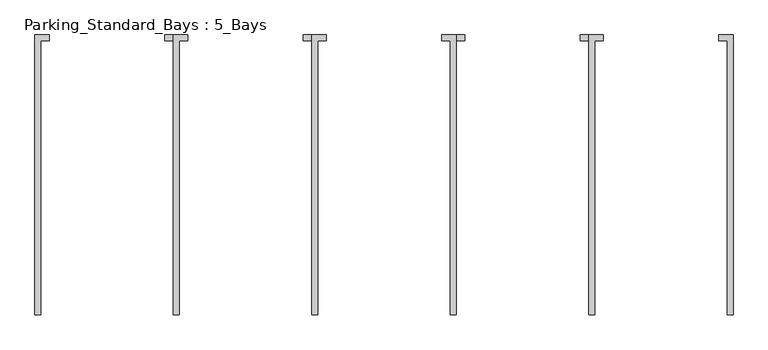
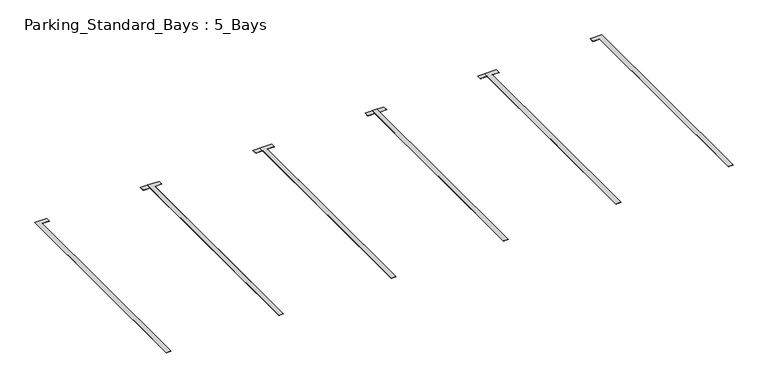
"""IFC4 building model written with IfcOpenShell, lengths in millimetres: proxy geometry, Parking_Standard_Bays : 5_Bays."""

from ifc_helpers import new_model, si_unit, origin, origin_with_axes, place, context, project, spatial, polyline, outline, extrude, source, transform, mapped, element, save


def parking_standard_bays_5_bays_00e1b54b(model_context):
    return source(origin(), model_context, "Body", "SweptSolid", [
        extrude(outline(polyline([(11950.0, 0.0), (11950.0, 4750.0), (11800.0, 4750.0), (11800.0, 4850.0), (12050.0, 4850.0), (12050.0, 0.0), (11950.0, 0.0)])), origin_with_axes(), (0.0, 0.0, 1.0), 3.175),
        extrude(outline(polyline([(9550.0, 0.0), (9550.0, 4850.0), (9800.0, 4850.0), (9800.0, 4750.0), (9650.0, 4750.0), (9650.0, 0.0), (9550.0, 0.0)])), origin_with_axes(), (0.0, 0.0, 1.0), 3.175),
        extrude(outline(polyline([(7150.0, 0.0), (7150.0, 4750.0), (7000.0, 4750.0), (7000.0, 4850.0), (7250.0, 4850.0), (7250.0, 0.0), (7150.0, 0.0)])), origin_with_axes(), (0.0, 0.0, 1.0), 3.175),
        extrude(outline(polyline([(4750.0, 0.0), (4750.0, 4850.0), (5000.0, 4850.0), (5000.0, 4750.0), (4850.0, 4750.0), (4850.0, 0.0), (4750.0, 0.0)])), origin_with_axes(), (0.0, 0.0, 1.0), 3.175),
        extrude(outline(polyline([(4750.0, 0.0), (4750.0, 4750.0), (4600.0, 4750.0), (4600.0, 4850.0), (4850.0, 4850.0), (4850.0, 0.0), (4750.0, 0.0)])), origin_with_axes(), (0.0, 0.0, 1.0), 3.175),
        extrude(outline(polyline([(2350.0, 0.0), (2350.0, 4850.0), (2600.0, 4850.0), (2600.0, 4750.0), (2450.0, 4750.0), (2450.0, 0.0), (2350.0, 0.0)])), origin_with_axes(), (0.0, 0.0, 1.0), 3.175),
        extrude(outline(polyline([(9550.0, 0.0), (9550.0, 4750.0), (9400.0, 4750.0), (9400.0, 4850.0), (9650.0, 4850.0), (9650.0, 0.0), (9550.0, 0.0)])), origin_with_axes(), (0.0, 0.0, 1.0), 3.175),
        extrude(outline(polyline([(7150.0, 0.0), (7150.0, 4850.0), (7400.0, 4850.0), (7400.0, 4750.0), (7250.0, 4750.0), (7250.0, 0.0), (7150.0, 0.0)])), origin_with_axes(), (0.0, 0.0, 1.0), 3.175),
        extrude(outline(polyline([(2350.0, 0.0), (2350.0, 4750.0), (2200.0, 4750.0), (2200.0, 4850.0), (2450.0, 4850.0), (2450.0, 0.0), (2350.0, 0.0)])), origin_with_axes(), (0.0, 0.0, 1.0), 3.175),
        extrude(outline(polyline([(-50.0, 0.0), (-50.0, 4850.0), (200.0, 4850.0), (200.0, 4750.0), (50.0, 4750.0), (50.0, 0.0), (-50.0, 0.0)])), origin_with_axes(), (0.0, 0.0, 1.0), 3.175),
    ])


if __name__ == "__main__":
    model = new_model("IFC4")
    model_context = context("Model", 3, world=origin())
    ifc_project = project(units=[si_unit("LENGTHUNIT", "METRE", prefix="MILLI")], contexts=[model_context])
    site = spatial("IfcSite", under=ifc_project)
    building = spatial("IfcBuilding", under=site)
    placement = place(None, origin())
    parking_standard_bays_5_bays_shape = parking_standard_bays_5_bays_00e1b54b(model_context)
    element("IfcBuildingElementProxy", 1, Name="Parking_Standard_Bays : 5_Bays", ObjectType="Parking_Standard_Bays : 5_Bays", at=placement, inside=building, context=model_context, shape_type="MappedRepresentation", body=[
        mapped(parking_standard_bays_5_bays_shape, transform((0.0, 0.0, 0.0), x_axis=(1.0, 0.0, 0.0), y_axis=(0.0, 1.0, 0.0), z_axis=(0.0, 0.0, 1.0))),
    ])
    save(model, "model.ifc")

# Revit data of these elements
# Type "Parking_Standard_Bays : 5_Bays"
#   Keynote = "Q22/185"
#   Length [instance default] = 14400 mm
#   Bay Width = 2400 mm
#   Bay Length = 4800 mm
#   No of Bays in Array [instance default] = 5
#   No of Bays [instance default] = 6
#   Material - White Lining = Paint - White Lining
# Element 1 (IfcBuildingElementProxy, "Parking_Standard_Bays : 5_Bays")
#   Length = 12000 mm
#   No of Bays in Array = 4
#   No of Bays = 5
#   Materials on its faces: "Paint - White Lining"
# Materials
#   "Paint - White Lining": class "Paint", colour RGB 239 247 247, transparency 0
